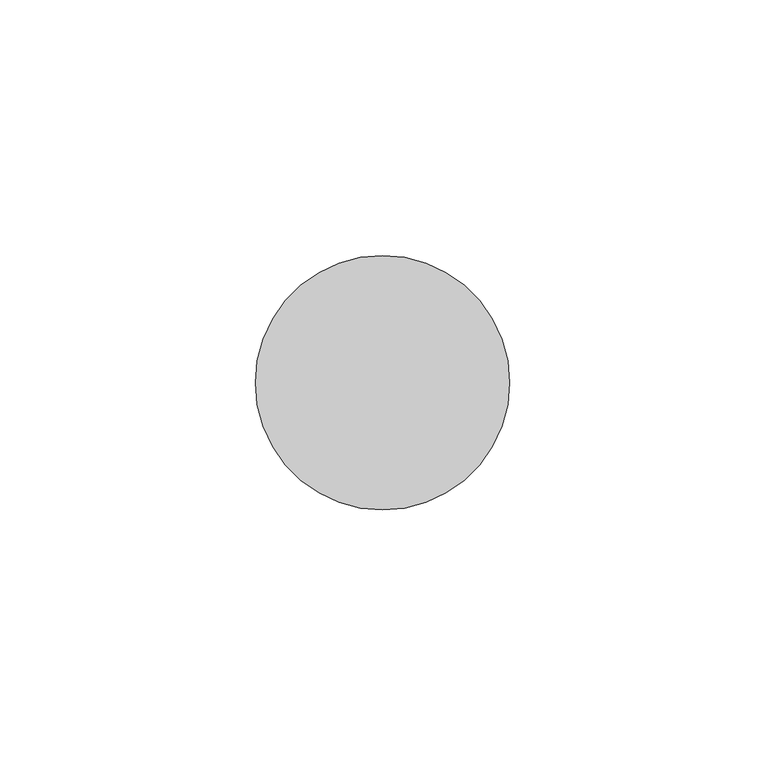
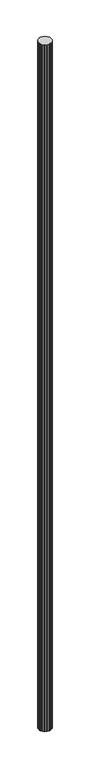
"""IFC4 building model written with IfcOpenShell, lengths in millimetres: proxy geometry, 0_3d_modell."""

import ifcopenshell
import ifcopenshell.guid

model = None  # the IFC model being written
_history = None  # IfcOwnerHistory: only IFC2X3 demands one
_inside = {}  # id of a spatial element -> (the spatial element, [elements in it])
_under = {}  # id of a project, library or spatial element -> (it, [spatial elements below it])
_declared = {}  # id of a project -> (the project, [libraries it declares])
_typed = {}  # id of a type object -> (the type object, [elements of that type])
_made_of = {}  # id of a material, layer set ... -> (it, [elements and type objects made of it])


def new_model(schema):
    """Start an empty IFC model of exactly this schema.

    Asked for "IFC4X3", IfcOpenShell would pick the latest addendum, in which some entities
    have other attributes; the version numbers below select the first issue.
    IFC2X3 requires an IfcOwnerHistory on every rooted entity: one is made here for all.
    """
    global model, _history
    if schema == "IFC4X3":
        model = ifcopenshell.file(schema_version=(4, 3, 0, 0))
    else:
        model = ifcopenshell.file(schema=schema)
    _inside.clear()
    _under.clear()
    _declared.clear()
    _typed.clear()
    _made_of.clear()
    _history = None
    if model.schema == "IFC2X3":
        org = make("IfcOrganization", Name="unknown")
        user = make(
            "IfcPersonAndOrganization",
            ThePerson=make("IfcPerson", FamilyName="unknown"),
            TheOrganization=org,
        )
        app = make(
            "IfcApplication",
            ApplicationDeveloper=org,
            Version="unknown",
            ApplicationFullName="unknown",
            ApplicationIdentifier="unknown",
        )
        _history = make(
            "IfcOwnerHistory",
            OwningUser=user,
            OwningApplication=app,
            ChangeAction="ADDED",
            CreationDate=0,
        )
    return model


def make(cls, **values):
    """One entity of the class cls with the attributes given. An attribute that is None is left unset."""
    return model.create_entity(
        cls, **{name: value for name, value in values.items() if value is not None}
    )


def rooted(cls, **values):
    """An entity with a GlobalId (a new one), such as an element, a storey or a relation."""
    return make(cls, GlobalId=ifcopenshell.guid.new(), OwnerHistory=_history, **values)


def si_unit(unit_type, name, prefix=None):
    """IfcSIUnit, for example si_unit("LENGTHUNIT", "METRE", prefix="MILLI")."""
    return make("IfcSIUnit", UnitType=unit_type, Prefix=prefix, Name=name)


def assignment(units):
    """IfcUnitAssignment: the units of a project."""
    return None if units is None else make("IfcUnitAssignment", Units=units)


def point(xyz):
    """IfcCartesianPoint."""
    return None if xyz is None else make("IfcCartesianPoint", Coordinates=xyz)


def direction(xyz):
    """IfcDirection."""
    return None if xyz is None else make("IfcDirection", DirectionRatios=xyz)


def frame(location, z_axis=None, x_axis=None):
    """IfcAxis2Placement3D, a coordinate frame: its origin and axes. An axis left out is left unset."""
    return make(
        "IfcAxis2Placement3D",
        Location=point(location),
        Axis=direction(z_axis),
        RefDirection=direction(x_axis),
    )


def origin():
    """The frame at (0, 0, 0) with its axes left unset."""
    return frame((0.0, 0.0, 0.0))


def origin_with_axes():
    """The frame at (0, 0, 0) with the z axis (0, 0, 1) and the x axis (1, 0, 0) written out."""
    return frame((0.0, 0.0, 0.0), z_axis=(0.0, 0.0, 1.0), x_axis=(1.0, 0.0, 0.0))


def place(relative_to, where):
    """IfcLocalPlacement: puts the frame where relative to a parent placement (None: the world)."""
    return make(
        "IfcLocalPlacement", PlacementRelTo=relative_to, RelativePlacement=where
    )


def context(
    kind, dimensions, precision=None, world=None, true_north=None, identifier=None
):
    """IfcGeometricRepresentationContext, for example the 3D "Model" context."""
    return make(
        "IfcGeometricRepresentationContext",
        ContextIdentifier=identifier,
        ContextType=kind,
        CoordinateSpaceDimension=dimensions,
        Precision=precision,
        WorldCoordinateSystem=world,
        TrueNorth=true_north,
    )


def project(units=None, contexts=None):
    """IfcProject with its units and contexts."""
    return rooted(
        "IfcProject",
        Name="project",
        RepresentationContexts=contexts,
        UnitsInContext=assignment(units),
    )


def spatial(cls, under=None, at=None, **own):
    """A site, building, storey or space (cls), placed at a placement, below another one or the project."""
    s = rooted(cls, ObjectPlacement=at, **own)
    if under is not None:
        _under.setdefault(under.id(), (under, []))[1].append(s)
    return s


def polyline(points):
    """IfcPolyline through the points."""
    return make("IfcPolyline", Points=[point(p) for p in points])


def outline(outer, holes=None, kind="AREA"):
    """IfcArbitraryClosedProfileDef: a profile drawn as a closed curve; with holes, ...WithVoids."""
    if holes is None:
        return make("IfcArbitraryClosedProfileDef", ProfileType=kind, OuterCurve=outer)
    return make(
        "IfcArbitraryProfileDefWithVoids",
        ProfileType=kind,
        OuterCurve=outer,
        InnerCurves=holes,
    )


def extrude(swept, where, along, depth):
    """IfcExtrudedAreaSolid: the profile swept, set in the frame where, extruded along a direction by depth."""
    return make(
        "IfcExtrudedAreaSolid",
        SweptArea=swept,
        Position=where,
        ExtrudedDirection=direction(along),
        Depth=depth,
    )


def shape(context_of_items, identifier, shape_type, items):
    """IfcShapeRepresentation: the items that make up one representation, for example the "Body"."""
    return make(
        "IfcShapeRepresentation",
        ContextOfItems=context_of_items,
        RepresentationIdentifier=identifier,
        RepresentationType=shape_type,
        Items=items,
    )


def source(mapping_origin, context_of_items, identifier, shape_type, items):
    """IfcRepresentationMap: a shape defined once, which mapped items show again and again."""
    return make(
        "IfcRepresentationMap",
        MappingOrigin=mapping_origin,
        MappedRepresentation=shape(context_of_items, identifier, shape_type, items),
    )


def transform(
    local_origin,
    x_axis=None,
    y_axis=None,
    z_axis=None,
    scale=None,
    scale2=None,
    scale3=None,
    uniform=True,
):
    """IfcCartesianTransformationOperator3D, or its non-uniform kind. x_axis, y_axis, z_axis: its Axis1, 2, 3."""
    if uniform:
        return make(
            "IfcCartesianTransformationOperator3D",
            Axis1=direction(x_axis),
            Axis2=direction(y_axis),
            LocalOrigin=point(local_origin),
            Scale=scale,
            Axis3=direction(z_axis),
        )
    return make(
        "IfcCartesianTransformationOperator3DnonUniform",
        Axis1=direction(x_axis),
        Axis2=direction(y_axis),
        LocalOrigin=point(local_origin),
        Scale=scale,
        Axis3=direction(z_axis),
        Scale2=scale2,
        Scale3=scale3,
    )


def mapped(mapping_source, mapping_target):
    """IfcMappedItem: shows the shape of a source again, moved by a transform."""
    return make(
        "IfcMappedItem", MappingSource=mapping_source, MappingTarget=mapping_target
    )


def made_of(thing, what):
    """Note that an element or type object is made of a material, layer set ...; save() writes the relation."""
    if what is not None:
        _made_of.setdefault(what.id(), (what, []))[1].append(thing)
    return thing


def element(
    cls,
    number,
    at=None,
    inside=None,
    cuts=None,
    type_object=None,
    material=None,
    context=None,
    identifier="Body",
    shape_type=None,
    held_by="IfcProductDefinitionShape",
    body=None,
    shapes=None,
    **own,
):
    """One element of the class cls, such as IfcWall. Its Tag is "e" and its number.

    at: its placement. inside: the storey or other place that contains it. cuts: it is an
    opening in that element (IfcRelVoidsElement). A single representation is given by context,
    identifier, shape_type and body (its items); several are given by shapes. held_by: the class
    of the entity that holds the representations. save() writes the other relations.
    """
    e = rooted(cls, Tag="e%d" % number, ObjectPlacement=at, **own)
    if body is not None:
        shapes = [shape(context, identifier, shape_type, body)]
    if shapes is not None:
        e.Representation = make(held_by, Representations=shapes)
    if inside is not None:
        _inside.setdefault(inside.id(), (inside, []))[1].append(e)
    if cuts is not None:
        rooted(
            "IfcRelVoidsElement", RelatingBuildingElement=cuts, RelatedOpeningElement=e
        )
    if type_object is not None:
        _typed.setdefault(type_object.id(), (type_object, []))[1].append(e)
    return made_of(e, material)


def aggregate(whole, parts):
    """IfcRelAggregates: a whole, such as a stair, and the parts it consists of."""
    return rooted("IfcRelAggregates", RelatingObject=whole, RelatedObjects=parts)


def save(model, path):
    """Write the relations noted so far, then the file.

    IfcRelAggregates (storeys below a building ...), IfcRelContainedInSpatialStructure (elements
    in a storey), IfcRelDefinesByType, IfcRelAssociatesMaterial and IfcRelDeclares: one each for
    every whole, place, type object, material and project.
    """
    for whole, parts in _under.values():
        aggregate(whole, parts)
    for where, things in _inside.values():
        rooted(
            "IfcRelContainedInSpatialStructure",
            RelatedElements=things,
            RelatingStructure=where,
        )
    for kind, things in _typed.values():
        rooted("IfcRelDefinesByType", RelatedObjects=things, RelatingType=kind)
    for what, things in _made_of.values():
        rooted("IfcRelAssociatesMaterial", RelatedObjects=things, RelatingMaterial=what)
    for by, libraries in _declared.values():
        rooted("IfcRelDeclares", RelatingContext=by, RelatedDefinitions=libraries)
    model.write(path)


def generic_models_b6edaf92(model_context):
    return source(origin(), model_context, "Body", "SweptSolid", [
        extrude(outline(polyline([(49.5185707, 29.3232855), (49.8968091, 25.0), (49.5185707, 20.6767145), (48.3953478, 16.4847898), (46.5612692, 12.5515954), (44.0720623, 8.9966396), (41.0033604, 5.9279377), (37.4484046, 3.4387308), (33.5152102, 1.6046522), (29.3232855, 0.4814293), (25.0, 0.1031909), (20.6767145, 0.4814293), (16.4847898, 1.6046522), (12.5515954, 3.4387308), (8.9966396, 5.9279377), (5.9279377, 8.9966396), (3.4387308, 12.5515954), (1.6046522, 16.4847898), (0.4814293, 20.6767145), (0.1031909, 25.0), (0.4814293, 29.3232855), (1.6046522, 33.5152102), (3.4387308, 37.4484046), (5.9279377, 41.0033604), (8.9966396, 44.0720623), (12.5515954, 46.5612692), (16.4847898, 48.3953478), (20.6767145, 49.5185707), (25.0, 49.8968091), (29.3232855, 49.5185707), (33.5152102, 48.3953478), (37.4484046, 46.5612692), (41.0033604, 44.0720623), (44.0720623, 41.0033604), (46.5612692, 37.4484046), (48.3953478, 33.5152102), (49.5185707, 29.3232855)])), origin_with_axes(), (0.0, 0.0, 1.0), 2855.0),
    ])


if __name__ == "__main__":
    model = new_model("IFC4")
    model_context = context("Model", 3, world=origin())
    ifc_project = project(units=[si_unit("LENGTHUNIT", "METRE", prefix="MILLI")], contexts=[model_context])
    site = spatial("IfcSite", under=ifc_project)
    building = spatial("IfcBuilding", under=site)
    placement = place(None, origin())
    generic_models_shape = generic_models_b6edaf92(model_context)
    element("IfcBuildingElementProxy", 1, Name="0_3d_modell", ObjectType="0_3d_modell", at=placement, inside=building, context=model_context, shape_type="MappedRepresentation", body=[
        mapped(generic_models_shape, transform((0.0, 0.0, 0.0), x_axis=(1.0, 0.0, 0.0), y_axis=(0.0, 1.0, 0.0), z_axis=(0.0, 0.0, 1.0))),
    ])
    save(model, "model.ifc")

# Revit data of these elements
# Element 1 (IfcBuildingElementProxy, "0_3d_modell")
#   Materials on its faces: "alu"
# Materials
#   "alu": class "Unassigned", colour RGB 219 219 219, transparency 0
